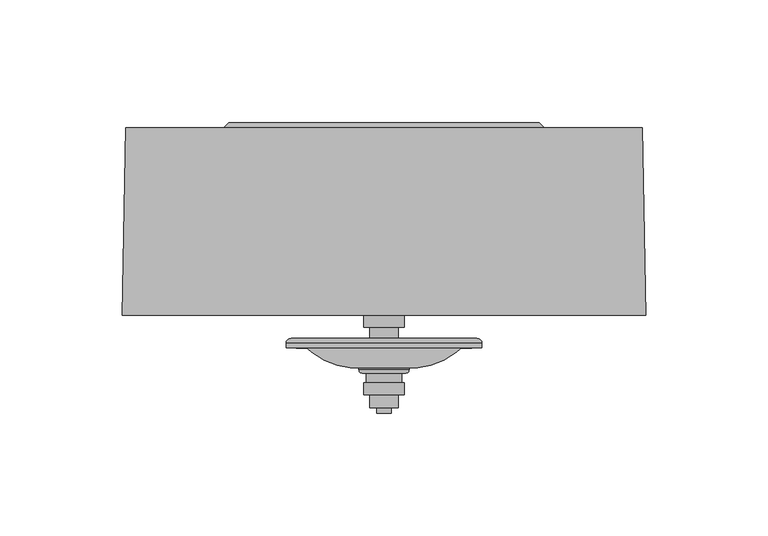
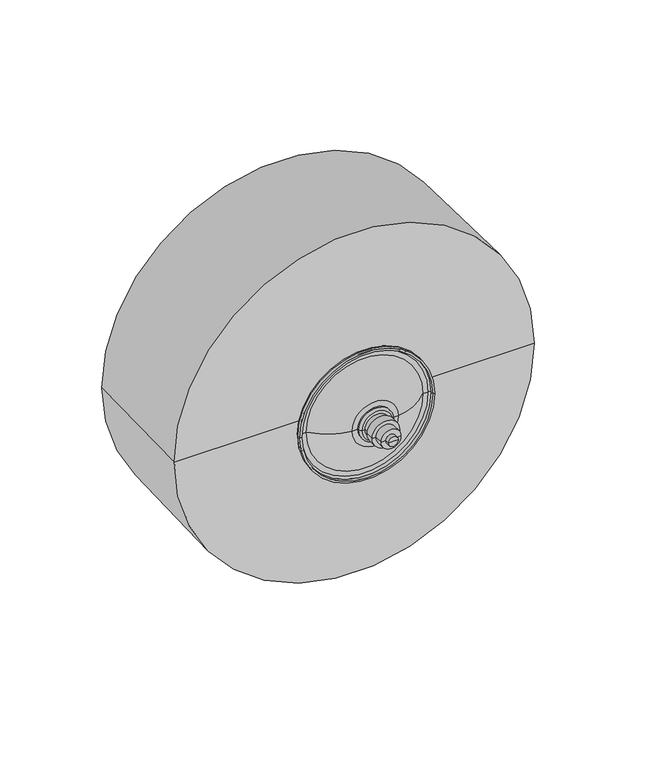
"""IFC4 building model written with IfcOpenShell, lengths in millimetres: proxy geometry, BVNO 50 4L : BVNO 50 4L."""

from ifc_helpers import new_model, si_unit, point, frame, origin, place, context, project, spatial, polyline, circle_curve, ellipse_curve, trimmed, source, transform, mapped, element, save
from ifc_brep_helpers import plane_surface, cylinder_surface, revolved_surface, spline_curve, advanced_brep


def mechanical_equipment_c477e944(model_context):
    return source(origin(), model_context, "Body", "AdvancedBrep", [
        advanced_brep(
        [(121.9974459, -0.199999, 2400.0), (128.0025541, -0.199999, 2400.0), (128.0025541, -2.4999994, 2400.0), (121.9974459, -2.4999994, 2400.0), (119.1058972, -0.199999, 2400.0), (130.8941028, -0.199999, 2400.0), (119.1058972, 4.9999993, 2400.0), (130.8941028, 4.9999993, 2400.0), (116.7764643, 4.9999993, 2400.0), (133.2235357, 4.9999993, 2400.0), (116.7764643, 10.0000007, 2400.0), (133.2235357, 10.0000007, 2400.0), (117.7564219, 10.0000007, 2400.0), (132.2435781, 10.0000007, 2400.0), (117.7564219, 13.8000004, 2400.0), (132.2435781, 13.8000004, 2400.0), (116.0662237, 13.8000004, 2400.0), (133.9337763, 13.8000004, 2400.0), (114.7691944, 15.1302816, 2400.0), (135.2308056, 15.1302816, 2400.0), (114.7691944, 15.9854344, 2400.0), (135.2308056, 15.9854344, 2400.0), (111.2784266, 15.9854344, 2400.0), (138.7215734, 15.9854344, 2400.0), (90.472179, 26.7999995, 2400.0), (159.527821, 26.7999995, 2400.0), (87.519154, 26.7999995, 2400.0), (162.480846, 26.7999995, 2400.0), (86.2128962, 25.9940284, 2400.0), (163.7871038, 25.9940284, 2400.0), (86.2128962, 24.0999996, 2400.0), (163.7871038, 24.0999996, 2400.0), (85.0392013, 24.0999996, 2400.0), (164.9607987, 24.0999996, 2400.0), (85.0392013, 25.9940284, 2400.0), (164.9607987, 25.9940284, 2400.0), (87.0451729, 28.0, 2400.0), (162.9548271, 28.0, 2400.0), (119.1058972, 28.0, 2400.0), (130.8941028, 28.0, 2400.0), (119.1058972, 32.5000002, 2400.0), (130.8941028, 32.5000002, 2400.0), (116.7764643, 32.5000002, 2400.0), (133.2235357, 32.5000002, 2400.0), (116.7764643, 37.4999999, 2400.0), (133.2235357, 37.4999999, 2400.0), (18.250711, 37.4999999, 2400.0), (231.749289, 37.4999999, 2400.0), (19.5859291, 113.9945916, 2400.0), (230.4140709, 113.9945916, 2400.0), (59.5859291, 113.9945916, 2400.0), (190.4140709, 113.9945916, 2400.0), (61.724849, 116.1335115, 2400.0), (188.275151, 116.1335115, 2400.0), (125.0, 116.1335115, 2400.0), (125.0, -2.4999994, 2400.0)],
        [
            (0, 1, circle_curve(frame((125.0, -0.199999, 2400.0), z_axis=(0.0, -1.0, 0.0), x_axis=(1.0, 0.0, 0.0)), 3.0025541)),
            (1, 2),
            (2, 3, circle_curve(frame((125.0, -2.4999994, 2400.0), z_axis=(0.0, 1.0, 0.0), x_axis=(1.0, 0.0, 0.0)), 3.0025541)),
            (3, 0),
            (1, 0, circle_curve(frame((125.0, -0.199999, 2400.0), z_axis=(0.0, -1.0, 0.0), x_axis=(1.0, 0.0, 0.0)), 3.0025541)),
            (3, 2, circle_curve(frame((125.0, -2.4999994, 2400.0), z_axis=(0.0, 1.0, 0.0), x_axis=(1.0, 0.0, 0.0)), 3.0025541)),
            (4, 5, circle_curve(frame((125.0, -0.199999, 2400.0), z_axis=(0.0, -1.0, 0.0), x_axis=(1.0, 0.0, 0.0)), 5.8941028)),
            (5, 1),
            (0, 4),
            (5, 4, circle_curve(frame((125.0, -0.199999, 2400.0), z_axis=(0.0, -1.0, 0.0), x_axis=(1.0, 0.0, 0.0)), 5.8941028)),
            (6, 7, circle_curve(frame((125.0, 4.9999993, 2400.0), z_axis=(0.0, -1.0, 0.0), x_axis=(1.0, 0.0, 0.0)), 5.8941028)),
            (7, 5),
            (4, 6),
            (7, 6, circle_curve(frame((125.0, 4.9999993, 2400.0), z_axis=(0.0, -1.0, 0.0), x_axis=(1.0, 0.0, 0.0)), 5.8941028)),
            (8, 9, circle_curve(frame((125.0, 4.9999993, 2400.0), z_axis=(0.0, -1.0, 0.0), x_axis=(1.0, 0.0, 0.0)), 8.2235357)),
            (9, 7),
            (6, 8),
            (9, 8, circle_curve(frame((125.0, 4.9999993, 2400.0), z_axis=(0.0, -1.0, 0.0), x_axis=(1.0, 0.0, 0.0)), 8.2235357)),
            (10, 11, circle_curve(frame((125.0, 10.0000007, 2400.0), z_axis=(0.0, -1.0, 0.0), x_axis=(1.0, 0.0, 0.0)), 8.2235357)),
            (11, 9),
            (8, 10),
            (11, 10, circle_curve(frame((125.0, 10.0000007, 2400.0), z_axis=(0.0, -1.0, 0.0), x_axis=(1.0, 0.0, 0.0)), 8.2235357)),
            (12, 13, circle_curve(frame((125.0, 10.0000007, 2400.0), z_axis=(0.0, -1.0, 0.0), x_axis=(1.0, 0.0, 0.0)), 7.2435781)),
            (13, 11),
            (10, 12),
            (13, 12, circle_curve(frame((125.0, 10.0000007, 2400.0), z_axis=(0.0, -1.0, 0.0), x_axis=(1.0, 0.0, 0.0)), 7.2435781)),
            (14, 15, circle_curve(frame((125.0, 13.8000004, 2400.0), z_axis=(0.0, -1.0, 0.0), x_axis=(1.0, 0.0, 0.0)), 7.2435781)),
            (15, 13),
            (12, 14),
            (15, 14, circle_curve(frame((125.0, 13.8000004, 2400.0), z_axis=(0.0, -1.0, 0.0), x_axis=(1.0, 0.0, 0.0)), 7.2435781)),
            (16, 17, circle_curve(frame((125.0, 13.8000004, 2400.0), z_axis=(0.0, -1.0, 0.0), x_axis=(1.0, 0.0, 0.0)), 8.9337763)),
            (17, 15),
            (14, 16),
            (17, 16, circle_curve(frame((125.0, 13.8000004, 2400.0), z_axis=(0.0, -1.0, 0.0), x_axis=(1.0, 0.0, 0.0)), 8.9337763)),
            (18, 19, circle_curve(frame((125.0, 15.1302816, 2400.0), z_axis=(0.0, -1.0, 0.0), x_axis=(1.0, 0.0, 0.0)), 10.2308056)),
            (19, 17, spline_curve(3, [(135.2308056, 15.1302816, 2400.0), (135.18031757, 14.408269131, 2400.0), (134.747974442, 13.964842091, 2400.0), (133.9337763, 13.8000004, 2400.0)], [4, 4], [0.0, 0.003825031864308585])),
            (16, 18, spline_curve(3, [(116.0662237, 13.8000004, 2400.0), (115.252025558, 13.964842091, 2400.0), (114.81968243, 14.408269131, 2400.0), (114.7691944, 15.1302816, 2400.0)], [4, 4], [0.0, 0.003825031864308585])),
            (19, 18, circle_curve(frame((125.0, 15.1302816, 2400.0), z_axis=(0.0, -1.0, 0.0), x_axis=(1.0, 0.0, 0.0)), 10.2308056)),
            (20, 21, circle_curve(frame((125.0, 15.9854344, 2400.0), z_axis=(0.0, -1.0, 0.0), x_axis=(1.0, 0.0, 0.0)), 10.2308056)),
            (21, 19),
            (18, 20),
            (21, 20, circle_curve(frame((125.0, 15.9854344, 2400.0), z_axis=(0.0, -1.0, 0.0), x_axis=(1.0, 0.0, 0.0)), 10.2308056)),
            (22, 23, circle_curve(frame((125.0, 15.9854344, 2400.0), z_axis=(0.0, -1.0, 0.0), x_axis=(1.0, 0.0, 0.0)), 13.7215734)),
            (23, 21),
            (20, 22),
            (23, 22, circle_curve(frame((125.0, 15.9854344, 2400.0), z_axis=(0.0, -1.0, 0.0), x_axis=(1.0, 0.0, 0.0)), 13.7215734)),
            (24, 25, circle_curve(frame((125.0, 26.7999995, 2400.0), z_axis=(0.0, -1.0, 0.0), x_axis=(1.0, 0.0, 0.0)), 34.527821)),
            (25, 23, spline_curve(3, [(159.527821, 26.7999995, 2400.0), (152.920328589, 20.192507089, 2400.0), (145.984912731, 16.587652064, 2400.0), (138.7215734, 15.9854344, 2400.0)], [4, 4], [0.0, 0.04037262450680565])),
            (22, 24, spline_curve(3, [(111.2784266, 15.9854344, 2400.0), (104.015087269, 16.587652064, 2400.0), (97.079671411, 20.192507089, 2400.0), (90.472179, 26.7999995, 2400.0)], [4, 4], [0.0, 0.04037262450680565])),
            (25, 24, circle_curve(frame((125.0, 26.7999995, 2400.0), z_axis=(0.0, -1.0, 0.0), x_axis=(1.0, 0.0, 0.0)), 34.527821)),
            (26, 27, circle_curve(frame((125.0, 26.7999995, 2400.0), z_axis=(0.0, -1.0, 0.0), x_axis=(1.0, 0.0, 0.0)), 37.480846)),
            (27, 25),
            (24, 26),
            (27, 26, circle_curve(frame((125.0, 26.7999995, 2400.0), z_axis=(0.0, -1.0, 0.0), x_axis=(1.0, 0.0, 0.0)), 37.480846)),
            (28, 29, circle_curve(frame((125.0, 25.9940284, 2400.0), z_axis=(0.0, -1.0, 0.0), x_axis=(1.0, 0.0, 0.0)), 38.7871038)),
            (29, 27, circle_curve(frame((162.7127782, 25.7143697, 2400.0), z_axis=(0.0, 0.0, 1.0), x_axis=(-1.0, 0.0, 0.0)), 1.1101281)),
            (26, 28, circle_curve(frame((87.2872218, 25.7143697, 2400.0), z_axis=(0.0, 0.0, 1.0), x_axis=(1.0, 0.0, 0.0)), 1.1101281)),
            (29, 28, circle_curve(frame((125.0, 25.9940284, 2400.0), z_axis=(0.0, -1.0, 0.0), x_axis=(1.0, 0.0, 0.0)), 38.7871038)),
            (30, 31, circle_curve(frame((125.0, 24.0999996, 2400.0), z_axis=(0.0, -1.0, 0.0), x_axis=(1.0, 0.0, 0.0)), 38.7871038)),
            (31, 29),
            (28, 30),
            (31, 30, circle_curve(frame((125.0, 24.0999996, 2400.0), z_axis=(0.0, -1.0, 0.0), x_axis=(1.0, 0.0, 0.0)), 38.7871038)),
            (32, 33, circle_curve(frame((125.0, 24.0999996, 2400.0), z_axis=(0.0, -1.0, 0.0), x_axis=(1.0, 0.0, 0.0)), 39.9607987)),
            (33, 31),
            (30, 32),
            (33, 32, circle_curve(frame((125.0, 24.0999996, 2400.0), z_axis=(0.0, -1.0, 0.0), x_axis=(1.0, 0.0, 0.0)), 39.9607987)),
            (34, 35, circle_curve(frame((125.0, 25.9940284, 2400.0), z_axis=(0.0, -1.0, 0.0), x_axis=(1.0, 0.0, 0.0)), 39.9607987)),
            (35, 33),
            (32, 34),
            (35, 34, circle_curve(frame((125.0, 25.9940284, 2400.0), z_axis=(0.0, -1.0, 0.0), x_axis=(1.0, 0.0, 0.0)), 39.9607987)),
            (36, 37, circle_curve(frame((125.0, 28.0, 2400.0), z_axis=(0.0, -1.0, 0.0), x_axis=(1.0, 0.0, 0.0)), 37.9548271)),
            (37, 35, circle_curve(frame((162.9548271, 25.9940284, 2400.0), z_axis=(0.0, 0.0, -1.0), x_axis=(-1.0, 0.0, 0.0)), 2.0059716)),
            (34, 36, circle_curve(frame((87.0451729, 25.9940284, 2400.0), z_axis=(0.0, 0.0, -1.0), x_axis=(1.0, 0.0, 0.0)), 2.0059716)),
            (37, 36, circle_curve(frame((125.0, 28.0, 2400.0), z_axis=(0.0, -1.0, 0.0), x_axis=(1.0, 0.0, 0.0)), 37.9548271)),
            (38, 39, circle_curve(frame((125.0, 28.0, 2400.0), z_axis=(0.0, -1.0, 0.0), x_axis=(1.0, 0.0, 0.0)), 5.8941028)),
            (39, 37),
            (36, 38),
            (39, 38, circle_curve(frame((125.0, 28.0, 2400.0), z_axis=(0.0, -1.0, 0.0), x_axis=(1.0, 0.0, 0.0)), 5.8941028)),
            (40, 41, circle_curve(frame((125.0, 32.5000002, 2400.0), z_axis=(0.0, -1.0, 0.0), x_axis=(1.0, 0.0, 0.0)), 5.8941028)),
            (41, 39),
            (38, 40),
            (41, 40, circle_curve(frame((125.0, 32.5000002, 2400.0), z_axis=(0.0, -1.0, 0.0), x_axis=(1.0, 0.0, 0.0)), 5.8941028)),
            (42, 43, circle_curve(frame((125.0, 32.5000002, 2400.0), z_axis=(0.0, -1.0, 0.0), x_axis=(1.0, 0.0, 0.0)), 8.2235357)),
            (43, 41),
            (40, 42),
            (43, 42, circle_curve(frame((125.0, 32.5000002, 2400.0), z_axis=(0.0, -1.0, 0.0), x_axis=(1.0, 0.0, 0.0)), 8.2235357)),
            (44, 45, circle_curve(frame((125.0, 37.4999999, 2400.0), z_axis=(0.0, -1.0, 0.0), x_axis=(1.0, 0.0, 0.0)), 8.2235357)),
            (45, 43),
            (42, 44),
            (45, 44, circle_curve(frame((125.0, 37.4999999, 2400.0), z_axis=(0.0, -1.0, 0.0), x_axis=(1.0, 0.0, 0.0)), 8.2235357)),
            (46, 47, circle_curve(frame((125.0, 37.4999999, 2400.0), z_axis=(0.0, -1.0, 0.0), x_axis=(1.0, 0.0, 0.0)), 106.749289)),
            (47, 45),
            (44, 46),
            (47, 46, circle_curve(frame((125.0, 37.4999999, 2400.0), z_axis=(0.0, -1.0, 0.0), x_axis=(1.0, 0.0, 0.0)), 106.749289)),
            (48, 49, circle_curve(frame((125.0, 113.9945916, 2400.0), z_axis=(0.0, -1.0, 0.0), x_axis=(1.0, 0.0, 0.0)), 105.4140709)),
            (49, 47),
            (46, 48),
            (49, 48, circle_curve(frame((125.0, 113.9945916, 2400.0), z_axis=(0.0, -1.0, 0.0), x_axis=(1.0, 0.0, 0.0)), 105.4140709)),
            (50, 51, circle_curve(frame((125.0, 113.9945916, 2400.0), z_axis=(0.0, -1.0, 0.0), x_axis=(1.0, 0.0, 0.0)), 65.4140709)),
            (51, 49),
            (48, 50),
            (51, 50, circle_curve(frame((125.0, 113.9945916, 2400.0), z_axis=(0.0, -1.0, 0.0), x_axis=(1.0, 0.0, 0.0)), 65.4140709)),
            (52, 53, circle_curve(frame((125.0, 116.1335115, 2400.0), z_axis=(0.0, -1.0, 0.0), x_axis=(1.0, 0.0, 0.0)), 63.275151)),
            (53, 51),
            (50, 52),
            (53, 52, circle_curve(frame((125.0, 116.1335115, 2400.0), z_axis=(0.0, -1.0, 0.0), x_axis=(1.0, 0.0, 0.0)), 63.275151)),
            (54, 53),
            (52, 54),
            (2, 55),
            (55, 3),
        ],
        [
            cylinder_surface(frame((125.0, -65.0, 2400.0), z_axis=(0.0, 1.0, 0.0), x_axis=(1.0, 0.0, 0.0)), 3.0025541),
            plane_surface(frame((125.0, -0.199999, 2400.0), z_axis=(0.0, -1.0, 0.0), x_axis=(1.0, 0.0, 0.0))),
            cylinder_surface(frame((125.0, -65.0, 2400.0), z_axis=(0.0, 1.0, 0.0), x_axis=(1.0, 0.0, 0.0)), 5.8941028),
            plane_surface(frame((125.0, 4.9999993, 2400.0), z_axis=(0.0, -1.0, 0.0), x_axis=(1.0, 0.0, 0.0))),
            cylinder_surface(frame((125.0, -65.0, 2400.0), z_axis=(0.0, 1.0, 0.0), x_axis=(1.0, 0.0, 0.0)), 8.2235357),
            plane_surface(frame((125.0, 10.0000007, 2400.0), z_axis=(0.0, 1.0, 0.0), x_axis=(1.0, 0.0, 0.0))),
            cylinder_surface(frame((125.0, -65.0, 2400.0), z_axis=(0.0, 1.0, 0.0), x_axis=(1.0, 0.0, 0.0)), 7.2435781),
            plane_surface(frame((125.0, 13.8000004, 2400.0), z_axis=(0.0, -1.0, 0.0), x_axis=(1.0, 0.0, 0.0))),
            revolved_surface(spline_curve(3, [(133.9337763, 13.8000004, 2400.0), (134.747974442, 13.964842091, 2400.0), (135.18031757, 14.408269131, 2400.0), (135.2308056, 15.1302816, 2400.0)], [4, 4], [0.0, 0.003825031864308585]), (125.0, -65.0, 2400.0), (0.0, 1.0, 0.0)),
            cylinder_surface(frame((125.0, -65.0, 2400.0), z_axis=(0.0, 1.0, 0.0), x_axis=(1.0, 0.0, 0.0)), 10.2308056),
            plane_surface(frame((125.0, 15.9854344, 2400.0), z_axis=(0.0, -1.0, 0.0), x_axis=(1.0, 0.0, 0.0))),
            revolved_surface(spline_curve(3, [(138.7215734, 15.9854344, 2400.0), (145.984912731, 16.587652064, 2400.0), (152.920328589, 20.192507089, 2400.0), (159.527821, 26.7999995, 2400.0)], [4, 4], [0.0, 0.04037262450680565]), (125.0, -65.0, 2400.0), (0.0, 1.0, 0.0)),
            plane_surface(frame((125.0, 26.7999995, 2400.0), z_axis=(0.0, -1.0, 0.0), x_axis=(1.0, 0.0, 0.0))),
            revolved_surface(trimmed(ellipse_curve(frame((162.7127782, 25.7143697, 2400.0), z_axis=(0.0, 0.0, -1.0), x_axis=(-1.0, 0.0, 0.0)), 1.1101281, 1.1101281), [point((162.480846, 26.7999995, 2400.0))], [point((163.7871038, 25.9940284, 2400.0))], True, "CARTESIAN"), (125.0, -65.0, 2400.0), (0.0, 1.0, 0.0)),
            revolved_surface(polyline([(163.7871038, 25.994028400000005, 2400.0), (163.7871038, 24.099999600000004, 2400.0)]), (125.0, -65.0, 2400.0), (0.0, 1.0, 0.0)),
            plane_surface(frame((125.0, 24.0999996, 2400.0), z_axis=(0.0, -1.0, 0.0), x_axis=(1.0, 0.0, 0.0))),
            cylinder_surface(frame((125.0, -65.0, 2400.0), z_axis=(0.0, 1.0, 0.0), x_axis=(1.0, 0.0, 0.0)), 39.9607987),
            revolved_surface(trimmed(ellipse_curve(frame((162.9548271, 25.9940284, 2400.0), z_axis=(0.0, 0.0, 1.0), x_axis=(-1.0, 0.0, 0.0)), 2.0059716, 2.0059716), [point((164.9607987, 25.9940284, 2400.0))], [point((162.9548271, 28.0, 2400.0))], True, "CARTESIAN"), (125.0, -65.0, 2400.0), (0.0, 1.0, 0.0)),
            plane_surface(frame((125.0, 28.0, 2400.0), z_axis=(0.0, 1.0, 0.0), x_axis=(1.0, 0.0, 0.0))),
            plane_surface(frame((125.0, 32.5000002, 2400.0), z_axis=(0.0, -1.0, 0.0), x_axis=(1.0, 0.0, 0.0))),
            plane_surface(frame((125.0, 37.4999999, 2400.0), z_axis=(0.0, -1.0, 0.0), x_axis=(1.0, 0.0, 0.0))),
            revolved_surface(polyline([(231.749289, 37.4999999, 2400.0), (230.4140709, 113.9945916, 2400.0)]), (125.0, -65.0, 2400.0), (0.0, 1.0, 0.0)),
            plane_surface(frame((125.0, 113.9945916, 2400.0), z_axis=(0.0, 1.0, 0.0), x_axis=(1.0, 0.0, 0.0))),
            revolved_surface(polyline([(190.4140709, 113.9945916, 2400.0), (188.275151, 116.1335115, 2400.0)]), (125.0, -65.0, 2400.0), (0.0, 1.0, 0.0)),
            plane_surface(frame((125.0, 116.1335115, 2400.0), z_axis=(0.0, 1.0, 0.0), x_axis=(1.0, 0.0, 0.0))),
            plane_surface(frame((125.0, -2.4999994, 2400.0), z_axis=(0.0, -1.0, 0.0), x_axis=(1.0, 0.0, 0.0))),
        ],
        [
            (0, [[1, 2, 3, 4]]),
            (0, [[5, -4, 6, -2]]),
            (1, [[7, 8, -1, 9]]),
            (1, [[10, -9, -5, -8]]),
            (2, [[11, 12, -7, 13]]),
            (2, [[14, -13, -10, -12]]),
            (3, [[15, 16, -11, 17]]),
            (3, [[18, -17, -14, -16]]),
            (4, [[19, 20, -15, 21]]),
            (4, [[22, -21, -18, -20]]),
            (5, [[23, 24, -19, 25]]),
            (5, [[26, -25, -22, -24]]),
            (6, [[27, 28, -23, 29]]),
            (6, [[30, -29, -26, -28]]),
            (7, [[31, 32, -27, 33]]),
            (7, [[34, -33, -30, -32]]),
            (8, [[35, 36, -31, 37]]),
            (8, [[38, -37, -34, -36]]),
            (9, [[39, 40, -35, 41]]),
            (9, [[42, -41, -38, -40]]),
            (10, [[43, 44, -39, 45]]),
            (10, [[46, -45, -42, -44]]),
            (11, [[47, 48, -43, 49]]),
            (11, [[50, -49, -46, -48]]),
            (12, [[51, 52, -47, 53]]),
            (12, [[54, -53, -50, -52]]),
            (13, [[55, 56, -51, 57]]),
            (13, [[58, -57, -54, -56]]),
            (14, [[59, 60, -55, 61]]),
            (14, [[62, -61, -58, -60]]),
            (15, [[63, 64, -59, 65]]),
            (15, [[66, -65, -62, -64]]),
            (16, [[67, 68, -63, 69]]),
            (16, [[70, -69, -66, -68]]),
            (17, [[71, 72, -67, 73]]),
            (17, [[74, -73, -70, -72]]),
            (18, [[75, 76, -71, 77]]),
            (18, [[78, -77, -74, -76]]),
            (2, [[79, 80, -75, 81]]),
            (2, [[82, -81, -78, -80]]),
            (19, [[83, 84, -79, 85]]),
            (19, [[86, -85, -82, -84]]),
            (4, [[87, 88, -83, 89]]),
            (4, [[90, -89, -86, -88]]),
            (20, [[91, 92, -87, 93]]),
            (20, [[94, -93, -90, -92]]),
            (21, [[95, 96, -91, 97]]),
            (21, [[98, -97, -94, -96]]),
            (22, [[99, 100, -95, 101]]),
            (22, [[102, -101, -98, -100]]),
            (23, [[103, 104, -99, 105]]),
            (23, [[106, -105, -102, -104]]),
            (24, [[107, -103, 108]]),
            (24, [[-108, -106, -107]]),
            (25, [[-3, 109, 110]]),
            (25, [[-6, -110, -109]]),
        ],
    ),
    ])


if __name__ == "__main__":
    model = new_model("IFC4")
    model_context = context("Model", 3, world=origin())
    ifc_project = project(units=[si_unit("LENGTHUNIT", "METRE", prefix="MILLI")], contexts=[model_context])
    site = spatial("IfcSite", under=ifc_project)
    building = spatial("IfcBuilding", under=site)
    placement = place(None, origin())
    mechanical_equipment_shape = mechanical_equipment_c477e944(model_context)
    element("IfcBuildingElementProxy", 1, Name="BVNO 50 4L : BVNO 50 4L", ObjectType="BVNO 50 4L : BVNO 50 4L", at=placement, inside=building, context=model_context, shape_type="MappedRepresentation", body=[
        mapped(mechanical_equipment_shape, transform((0.0, 0.0, 0.0), x_axis=(1.0, 0.0, 0.0), y_axis=(0.0, 1.0, 0.0), z_axis=(0.0, 0.0, 1.0))),
    ])
    save(model, "model.ifc")

# Revit data of these elements
# Type "BVNO 50 4L : BVNO 50 4L"
#   Model = "BVNO 50 4L"
#   FLANGE HEIGHT [instance default] = 2400 mm
#   Default Elevation = 0
